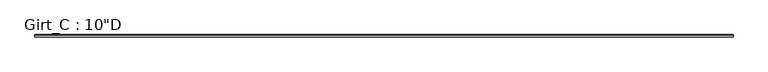
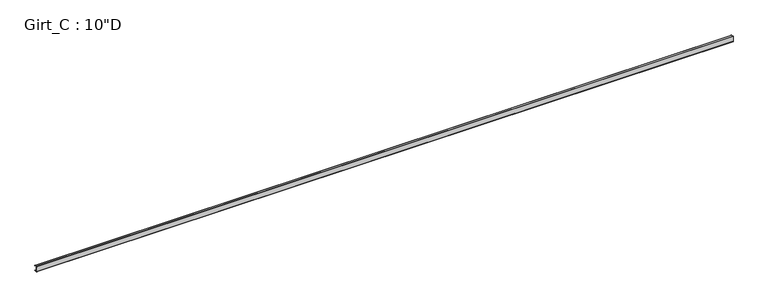
"""IFC4 building model written with IfcOpenShell, lengths in millimetres: beam geometry."""

from ifc_helpers import new_model, si_unit, point, frame, frame_2d, origin, place, context, project, spatial, polyline, circle_curve, trimmed, segment, composite_curve, outline, extrude, source, transform, mapped, element, save


def beam_2726e444(model_context):
    return source(origin(), model_context, "Body", "SweptSolid", [
        extrude(outline(composite_curve([segment(polyline([(87.5109375, 127.0), (99.7560415, 112.4068534), (97.6278742, 110.621109), (86.2154765, 124.221875), (3.3005807, 124.221875)]), True, "CONTINUOUS"), segment(trimmed(circle_curve(frame_2d((3.3741066, 122.2381931)), 1.9850441), [point((3.3005807, 124.221875))], [point((1.3890625, 122.2381931))], True, "CARTESIAN"), True, "CONTINUOUS"), segment(polyline([(1.3890625, 122.2381931), (1.3890625, -122.2389339)]), True, "CONTINUOUS"), segment(trimmed(circle_curve(frame_2d((3.3748024, -122.2389339)), 1.9857399), [point((1.3890625, -122.2389339))], [point((3.2694106, -124.221875))], True, "CARTESIAN"), True, "CONTINUOUS"), segment(polyline([(3.2694106, -124.221875), (86.2154765, -124.221875), (97.6510975, -110.5934327), (99.7792647, -112.379177), (87.5109375, -127.0), (3.3734375, -127.0)]), True, "CONTINUOUS"), segment(trimmed(circle_curve(frame_2d((3.3734375, -122.2375)), 4.7625), [point((3.3734375, -127.0))], [point((-1.3890625, -122.2375))], False, "CARTESIAN"), True, "CONTINUOUS"), segment(polyline([(-1.3890625, -122.2375), (-1.3890625, 122.2375)]), True, "CONTINUOUS"), segment(trimmed(circle_curve(frame_2d((3.3734375, 122.2375)), 4.7625), [point((-1.3890625, 122.2375))], [point((3.3734375, 127.0))], False, "CARTESIAN"), True, "CONTINUOUS"), segment(polyline([(3.3734375, 127.0), (87.5109375, 127.0)]), True, "CONTINUOUS")], self_intersect=False)), frame((-15567.025, 0.0, 0.0), z_axis=(1.0, 0.0, 0.0), x_axis=(0.0, 1.0, 0.0)), (0.0, 0.0, 1.0), 31083.25),
    ])


if __name__ == "__main__":
    model = new_model("IFC4")
    model_context = context("Model", 3, world=origin())
    ifc_project = project(units=[si_unit("LENGTHUNIT", "METRE", prefix="MILLI")], contexts=[model_context])
    site = spatial("IfcSite", under=ifc_project)
    building = spatial("IfcBuilding", under=site)
    placement = place(None, origin())
    beam_shape = beam_2726e444(model_context)
    element("IfcBeam", 1, ObjectType="Girt_C : 10\"D", at=placement, inside=building, context=model_context, shape_type="MappedRepresentation", body=[
        mapped(beam_shape, transform((0.0, 0.0, 0.0), x_axis=(1.0, 0.0, 0.0), y_axis=(0.0, 1.0, 0.0), z_axis=(0.0, 0.0, 1.0))),
    ])
    save(model, "model.ifc")

# Revit data of these elements
# Type "Girt_C : 10\"D"
#   half leg = 0' - 1 3/4"
#   Web_Thickness = 0' - 0 7/64"
#   Length [instance default] = 10' - 0"
#   Leg_1 = 0' - 3 1/2"
#   Height = 0' - 10"
#   Structural Material [instance default] = none
